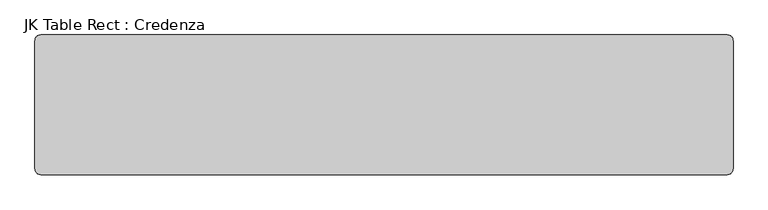
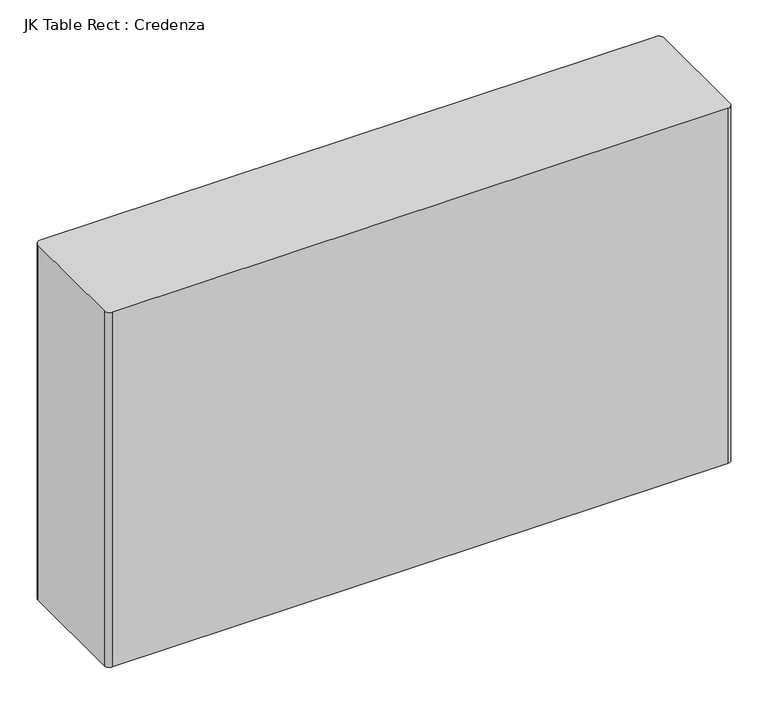
"""IFC4 building model written with IfcOpenShell, lengths in millimetres: furniture geometry, JK Table Rect : Credenza."""

import ifcopenshell
import ifcopenshell.guid

model = None  # the IFC model being written
_history = None  # IfcOwnerHistory: only IFC2X3 demands one
_inside = {}  # id of a spatial element -> (the spatial element, [elements in it])
_under = {}  # id of a project, library or spatial element -> (it, [spatial elements below it])
_declared = {}  # id of a project -> (the project, [libraries it declares])
_typed = {}  # id of a type object -> (the type object, [elements of that type])
_made_of = {}  # id of a material, layer set ... -> (it, [elements and type objects made of it])


def new_model(schema):
    """Start an empty IFC model of exactly this schema.

    Asked for "IFC4X3", IfcOpenShell would pick the latest addendum, in which some entities
    have other attributes; the version numbers below select the first issue.
    IFC2X3 requires an IfcOwnerHistory on every rooted entity: one is made here for all.
    """
    global model, _history
    if schema == "IFC4X3":
        model = ifcopenshell.file(schema_version=(4, 3, 0, 0))
    else:
        model = ifcopenshell.file(schema=schema)
    _inside.clear()
    _under.clear()
    _declared.clear()
    _typed.clear()
    _made_of.clear()
    _history = None
    if model.schema == "IFC2X3":
        org = make("IfcOrganization", Name="unknown")
        user = make(
            "IfcPersonAndOrganization",
            ThePerson=make("IfcPerson", FamilyName="unknown"),
            TheOrganization=org,
        )
        app = make(
            "IfcApplication",
            ApplicationDeveloper=org,
            Version="unknown",
            ApplicationFullName="unknown",
            ApplicationIdentifier="unknown",
        )
        _history = make(
            "IfcOwnerHistory",
            OwningUser=user,
            OwningApplication=app,
            ChangeAction="ADDED",
            CreationDate=0,
        )
    return model


def make(cls, **values):
    """One entity of the class cls with the attributes given. An attribute that is None is left unset."""
    return model.create_entity(
        cls, **{name: value for name, value in values.items() if value is not None}
    )


def rooted(cls, **values):
    """An entity with a GlobalId (a new one), such as an element, a storey or a relation."""
    return make(cls, GlobalId=ifcopenshell.guid.new(), OwnerHistory=_history, **values)


def si_unit(unit_type, name, prefix=None):
    """IfcSIUnit, for example si_unit("LENGTHUNIT", "METRE", prefix="MILLI")."""
    return make("IfcSIUnit", UnitType=unit_type, Prefix=prefix, Name=name)


def assignment(units):
    """IfcUnitAssignment: the units of a project."""
    return None if units is None else make("IfcUnitAssignment", Units=units)


def point(xyz):
    """IfcCartesianPoint."""
    return None if xyz is None else make("IfcCartesianPoint", Coordinates=xyz)


def direction(xyz):
    """IfcDirection."""
    return None if xyz is None else make("IfcDirection", DirectionRatios=xyz)


def frame(location, z_axis=None, x_axis=None):
    """IfcAxis2Placement3D, a coordinate frame: its origin and axes. An axis left out is left unset."""
    return make(
        "IfcAxis2Placement3D",
        Location=point(location),
        Axis=direction(z_axis),
        RefDirection=direction(x_axis),
    )


def frame_2d(location, x_axis=None):
    """IfcAxis2Placement2D, a coordinate frame in the plane: its origin and x axis."""
    return make(
        "IfcAxis2Placement2D", Location=point(location), RefDirection=direction(x_axis)
    )


def origin():
    """The frame at (0, 0, 0) with its axes left unset."""
    return frame((0.0, 0.0, 0.0))


def origin_with_axes():
    """The frame at (0, 0, 0) with the z axis (0, 0, 1) and the x axis (1, 0, 0) written out."""
    return frame((0.0, 0.0, 0.0), z_axis=(0.0, 0.0, 1.0), x_axis=(1.0, 0.0, 0.0))


def place(relative_to, where):
    """IfcLocalPlacement: puts the frame where relative to a parent placement (None: the world)."""
    return make(
        "IfcLocalPlacement", PlacementRelTo=relative_to, RelativePlacement=where
    )


def context(
    kind, dimensions, precision=None, world=None, true_north=None, identifier=None
):
    """IfcGeometricRepresentationContext, for example the 3D "Model" context."""
    return make(
        "IfcGeometricRepresentationContext",
        ContextIdentifier=identifier,
        ContextType=kind,
        CoordinateSpaceDimension=dimensions,
        Precision=precision,
        WorldCoordinateSystem=world,
        TrueNorth=true_north,
    )


def project(units=None, contexts=None):
    """IfcProject with its units and contexts."""
    return rooted(
        "IfcProject",
        Name="project",
        RepresentationContexts=contexts,
        UnitsInContext=assignment(units),
    )


def spatial(cls, under=None, at=None, **own):
    """A site, building, storey or space (cls), placed at a placement, below another one or the project."""
    s = rooted(cls, ObjectPlacement=at, **own)
    if under is not None:
        _under.setdefault(under.id(), (under, []))[1].append(s)
    return s


def polyline(points):
    """IfcPolyline through the points."""
    return make("IfcPolyline", Points=[point(p) for p in points])


def circle_curve(where, radius):
    """IfcCircle in the frame where."""
    return make("IfcCircle", Position=where, Radius=radius)


def trimmed(basis, trim1, trim2, sense, master):
    """IfcTrimmedCurve: the piece of a basis curve between two trims."""
    return make(
        "IfcTrimmedCurve",
        BasisCurve=basis,
        Trim1=trim1,
        Trim2=trim2,
        SenseAgreement=sense,
        MasterRepresentation=master,
    )


def segment(curve, same_sense, transition):
    """IfcCompositeCurveSegment."""
    return make(
        "IfcCompositeCurveSegment",
        Transition=transition,
        SameSense=same_sense,
        ParentCurve=curve,
    )


def composite_curve(segments, self_intersect=None):
    """IfcCompositeCurve: segments joined end to end."""
    return make("IfcCompositeCurve", Segments=segments, SelfIntersect=self_intersect)


def outline(outer, holes=None, kind="AREA"):
    """IfcArbitraryClosedProfileDef: a profile drawn as a closed curve; with holes, ...WithVoids."""
    if holes is None:
        return make("IfcArbitraryClosedProfileDef", ProfileType=kind, OuterCurve=outer)
    return make(
        "IfcArbitraryProfileDefWithVoids",
        ProfileType=kind,
        OuterCurve=outer,
        InnerCurves=holes,
    )


def extrude(swept, where, along, depth):
    """IfcExtrudedAreaSolid: the profile swept, set in the frame where, extruded along a direction by depth."""
    return make(
        "IfcExtrudedAreaSolid",
        SweptArea=swept,
        Position=where,
        ExtrudedDirection=direction(along),
        Depth=depth,
    )


def shape(context_of_items, identifier, shape_type, items):
    """IfcShapeRepresentation: the items that make up one representation, for example the "Body"."""
    return make(
        "IfcShapeRepresentation",
        ContextOfItems=context_of_items,
        RepresentationIdentifier=identifier,
        RepresentationType=shape_type,
        Items=items,
    )


def source(mapping_origin, context_of_items, identifier, shape_type, items):
    """IfcRepresentationMap: a shape defined once, which mapped items show again and again."""
    return make(
        "IfcRepresentationMap",
        MappingOrigin=mapping_origin,
        MappedRepresentation=shape(context_of_items, identifier, shape_type, items),
    )


def transform(
    local_origin,
    x_axis=None,
    y_axis=None,
    z_axis=None,
    scale=None,
    scale2=None,
    scale3=None,
    uniform=True,
):
    """IfcCartesianTransformationOperator3D, or its non-uniform kind. x_axis, y_axis, z_axis: its Axis1, 2, 3."""
    if uniform:
        return make(
            "IfcCartesianTransformationOperator3D",
            Axis1=direction(x_axis),
            Axis2=direction(y_axis),
            LocalOrigin=point(local_origin),
            Scale=scale,
            Axis3=direction(z_axis),
        )
    return make(
        "IfcCartesianTransformationOperator3DnonUniform",
        Axis1=direction(x_axis),
        Axis2=direction(y_axis),
        LocalOrigin=point(local_origin),
        Scale=scale,
        Axis3=direction(z_axis),
        Scale2=scale2,
        Scale3=scale3,
    )


def mapped(mapping_source, mapping_target):
    """IfcMappedItem: shows the shape of a source again, moved by a transform."""
    return make(
        "IfcMappedItem", MappingSource=mapping_source, MappingTarget=mapping_target
    )


def made_of(thing, what):
    """Note that an element or type object is made of a material, layer set ...; save() writes the relation."""
    if what is not None:
        _made_of.setdefault(what.id(), (what, []))[1].append(thing)
    return thing


def element(
    cls,
    number,
    at=None,
    inside=None,
    cuts=None,
    type_object=None,
    material=None,
    context=None,
    identifier="Body",
    shape_type=None,
    held_by="IfcProductDefinitionShape",
    body=None,
    shapes=None,
    **own,
):
    """One element of the class cls, such as IfcWall. Its Tag is "e" and its number.

    at: its placement. inside: the storey or other place that contains it. cuts: it is an
    opening in that element (IfcRelVoidsElement). A single representation is given by context,
    identifier, shape_type and body (its items); several are given by shapes. held_by: the class
    of the entity that holds the representations. save() writes the other relations.
    """
    e = rooted(cls, Tag="e%d" % number, ObjectPlacement=at, **own)
    if body is not None:
        shapes = [shape(context, identifier, shape_type, body)]
    if shapes is not None:
        e.Representation = make(held_by, Representations=shapes)
    if inside is not None:
        _inside.setdefault(inside.id(), (inside, []))[1].append(e)
    if cuts is not None:
        rooted(
            "IfcRelVoidsElement", RelatingBuildingElement=cuts, RelatedOpeningElement=e
        )
    if type_object is not None:
        _typed.setdefault(type_object.id(), (type_object, []))[1].append(e)
    return made_of(e, material)


def aggregate(whole, parts):
    """IfcRelAggregates: a whole, such as a stair, and the parts it consists of."""
    return rooted("IfcRelAggregates", RelatingObject=whole, RelatedObjects=parts)


def save(model, path):
    """Write the relations noted so far, then the file.

    IfcRelAggregates (storeys below a building ...), IfcRelContainedInSpatialStructure (elements
    in a storey), IfcRelDefinesByType, IfcRelAssociatesMaterial and IfcRelDeclares: one each for
    every whole, place, type object, material and project.
    """
    for whole, parts in _under.values():
        aggregate(whole, parts)
    for where, things in _inside.values():
        rooted(
            "IfcRelContainedInSpatialStructure",
            RelatedElements=things,
            RelatingStructure=where,
        )
    for kind, things in _typed.values():
        rooted("IfcRelDefinesByType", RelatedObjects=things, RelatingType=kind)
    for what, things in _made_of.values():
        rooted("IfcRelAssociatesMaterial", RelatedObjects=things, RelatingMaterial=what)
    for by, libraries in _declared.values():
        rooted("IfcRelDeclares", RelatingContext=by, RelatedDefinitions=libraries)
    model.write(path)


def jk_table_rect_credenza_ad9c788b(model_context):
    return source(origin(), model_context, "Body", "SweptSolid", [
        extrude(outline(composite_curve([segment(trimmed(circle_curve(frame_2d((687.3573665, 173.2455296)), 12.7), [point((687.3573665, 185.9455296))], [point((700.0573665, 173.2455296))], False, "CARTESIAN"), True, "CONTINUOUS"), segment(polyline([(700.0573665, 173.2455296), (700.0573665, -106.1544704)]), True, "CONTINUOUS"), segment(trimmed(circle_curve(frame_2d((687.3573665, -106.1544704)), 12.7), [point((700.0573665, -106.1544704))], [point((687.3573665, -118.8544704))], False, "CARTESIAN"), True, "CONTINUOUS"), segment(polyline([(687.3573665, -118.8544704), (-811.2426335, -118.8544704)]), True, "CONTINUOUS"), segment(trimmed(circle_curve(frame_2d((-811.2426335, -106.1544704)), 12.7), [point((-811.2426335, -118.8544704))], [point((-823.9426335, -106.1544704))], False, "CARTESIAN"), True, "CONTINUOUS"), segment(polyline([(-823.9426335, -106.1544704), (-823.9426335, 173.2455296)]), True, "CONTINUOUS"), segment(trimmed(circle_curve(frame_2d((-811.2426335, 173.2455296)), 12.7), [point((-823.9426335, 173.2455296))], [point((-811.2426335, 185.9455296))], False, "CARTESIAN"), True, "CONTINUOUS"), segment(polyline([(-811.2426335, 185.9455296), (687.3573665, 185.9455296)]), True, "CONTINUOUS")], self_intersect=False)), origin_with_axes(), (0.0, 0.0, 1.0), 914.4),
    ])


if __name__ == "__main__":
    model = new_model("IFC4")
    model_context = context("Model", 3, world=origin())
    ifc_project = project(units=[si_unit("LENGTHUNIT", "METRE", prefix="MILLI")], contexts=[model_context])
    site = spatial("IfcSite", under=ifc_project)
    building = spatial("IfcBuilding", under=site)
    placement = place(None, origin())
    jk_table_rect_credenza_shape = jk_table_rect_credenza_ad9c788b(model_context)
    element("IfcFurniture", 1, ObjectType="JK Table Rect : Credenza", at=placement, inside=building, context=model_context, shape_type="MappedRepresentation", body=[
        mapped(jk_table_rect_credenza_shape, transform((0.0, 0.0, 0.0), x_axis=(1.0, 0.0, 0.0), y_axis=(0.0, 1.0, 0.0), z_axis=(0.0, 0.0, 1.0))),
    ])
    save(model, "model.ifc")

# Revit data of these elements
# Type "JK Table Rect : Credenza"
#   Width = 5' - 0"
#   Height = 3' - 0"
#   Depth = 1' - 0"
#   Corner Radius = 0' - 0 1/2"
#   Status [instance default] = none
#   Default Elevation = 0
